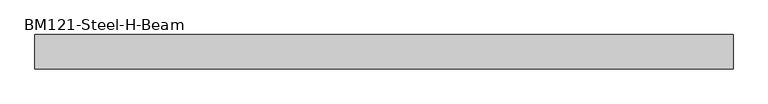
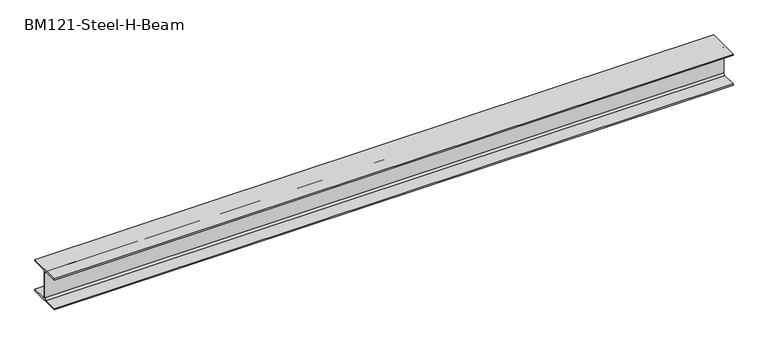
"""IFC4 building model written with IfcOpenShell, lengths in millimetres: beam geometry, BM121-Steel-H-Beam : BM121_H-294×302x12x12."""

from ifc_helpers import new_model, si_unit, point, frame, frame_2d, origin, place, context, project, spatial, polyline, circle_curve, trimmed, segment, composite_curve, outline, extrude, source, transform, mapped, element, save


def bm121_steel_h_beam_e2221314(model_context):
    return source(origin(), model_context, "Body", "SweptSolid", [
        extrude(outline(composite_curve([segment(polyline([(151.0, 147.0), (151.0, 135.0), (24.0, 135.0)]), True, "CONTINUOUS"), segment(trimmed(circle_curve(frame_2d((24.0, 117.0)), 18.0), [point((24.0, 135.0))], [point((6.0, 117.0))], True, "CARTESIAN"), True, "CONTINUOUS"), segment(polyline([(6.0, 117.0), (6.0, -117.0)]), True, "CONTINUOUS"), segment(trimmed(circle_curve(frame_2d((24.0, -117.0)), 18.0), [point((6.0, -117.0))], [point((24.0, -135.0))], True, "CARTESIAN"), True, "CONTINUOUS"), segment(polyline([(24.0, -135.0), (151.0, -135.0), (151.0, -147.0), (-151.0, -147.0), (-151.0, -135.0), (-24.0, -135.0)]), True, "CONTINUOUS"), segment(trimmed(circle_curve(frame_2d((-24.0, -117.0)), 18.0), [point((-24.0, -135.0))], [point((-6.0, -117.0))], True, "CARTESIAN"), True, "CONTINUOUS"), segment(polyline([(-6.0, -117.0), (-6.0, 117.0)]), True, "CONTINUOUS"), segment(trimmed(circle_curve(frame_2d((-24.0, 117.0)), 18.0), [point((-6.0, 117.0))], [point((-24.0, 135.0))], True, "CARTESIAN"), True, "CONTINUOUS"), segment(polyline([(-24.0, 135.0), (-151.0, 135.0), (-151.0, 147.0), (151.0, 147.0)]), True, "CONTINUOUS")], self_intersect=False)), frame((-3049.1486745, 0.0, 0.0), z_axis=(1.0, 0.0, 0.0), x_axis=(0.0, 1.0, 0.0)), (0.0, 0.0, 1.0), 6098.297349),
    ])


if __name__ == "__main__":
    model = new_model("IFC4")
    model_context = context("Model", 3, world=origin())
    ifc_project = project(units=[si_unit("LENGTHUNIT", "METRE", prefix="MILLI")], contexts=[model_context])
    site = spatial("IfcSite", under=ifc_project)
    building = spatial("IfcBuilding", under=site)
    placement = place(None, origin())
    bm121_steel_h_beam_shape = bm121_steel_h_beam_e2221314(model_context)
    element("IfcBeam", 1, ObjectType="BM121-Steel-H-Beam : BM121_H-294×302x12x12", at=placement, inside=building, context=model_context, shape_type="MappedRepresentation", body=[
        mapped(bm121_steel_h_beam_shape, transform((0.0, 0.0, 0.0), x_axis=(1.0, 0.0, 0.0), y_axis=(0.0, 1.0, 0.0), z_axis=(0.0, 0.0, 1.0))),
    ])
    save(model, "model.ifc")

# Revit data of these elements
# Type "BM121-Steel-H-Beam : BM121_H-294×302x12x12"
#   tw = 12 mm
#   tf = 12 mm
#   r = 18 mm
#   bf = 302 mm
#   Unit Weight = 84.50 kg/m
#   Surface Area = 1.7411 m²/m
#   Length [instance default] = 3000 mm
#   H = 294 mm
#   Sectional Area = 10770.0 cm²
